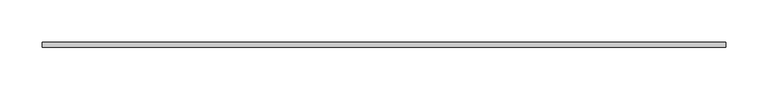
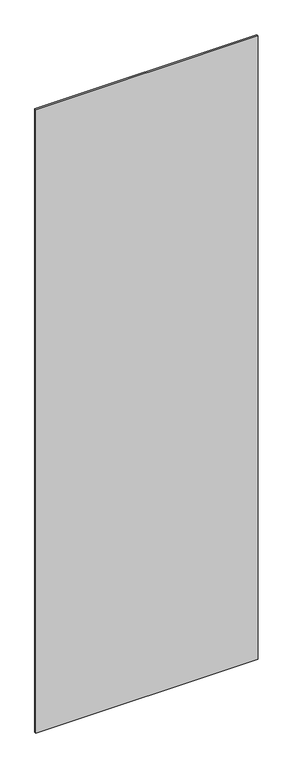
"""IFC4 building model written with IfcOpenShell, lengths in millimetres: proxy geometry, Window glass:Window glass:300352:Window glass:300352 : Window glass:Window glass:300352:300073:Window glass:300352:Window glass:300352 : Window glass:Window glass:300352:300073 : Window glass:Window glass:300352:Window glass:300352 : Window glass:Window glass:300352:300073:2 : Window glass:Window glass:300352:Window glass:300352 : Window glass:Window glass:300352:300073:Window glass:300352:Window glass:300352 : Window glass:Window glass:300352:300073 : Window glass:Window glass:300352:Window glass:300352 : Window glass:Window glass:300352:300073:300061."""

from ifc_helpers import new_model, si_unit, frame, origin, place, context, project, spatial, polyline, outline, extrude, source, transform, mapped, element, save


def generic_models_df3356e1(model_context):
    return source(origin(), model_context, "Body", "SweptSolid", [
        extrude(outline(polyline([(593690.1661787, -568062.3194464), (592877.9572692, -568062.3194464), (592877.9572692, -568055.9694464), (593690.1661787, -568055.9694464), (593690.1661787, -568062.3194464)])), frame((0.0, 0.0, 38.9089443), z_axis=(0.0, 0.0, 1.0), x_axis=(1.0, 0.0, 0.0)), (0.0, 0.0, 1.0), 2406.8704986),
    ])


if __name__ == "__main__":
    model = new_model("IFC4")
    model_context = context("Model", 3, world=origin())
    ifc_project = project(units=[si_unit("LENGTHUNIT", "METRE", prefix="MILLI")], contexts=[model_context])
    site = spatial("IfcSite", under=ifc_project)
    building = spatial("IfcBuilding", under=site)
    placement = place(None, origin())
    generic_models_shape = generic_models_df3356e1(model_context)
    element("IfcBuildingElementProxy", 1, Name="Window glass:Window glass:300352:Window glass:300352 : Window glass:Window glass:300352:300073:Window glass:300352:Window glass:300352 : Window glass:Window glass:300352:300073 : Window glass:Window glass:300352:Window glass:300352 : Window glass:Window glass:300352:300073:2 : Window glass:Window glass:300352:Window glass:300352 : Window glass:Window glass:300352:300073:Window glass:300352:Window glass:300352 : Window glass:Window glass:300352:300073 : Window glass:Window glass:300352:Window glass:300352 : Window glass:Window glass:300352:300073:300061", ObjectType="Window glass:Window glass:300352:Window glass:300352 : Window glass:Window glass:300352:300073:Window glass:300352:Window glass:300352 : Window glass:Window glass:300352:300073 : Window glass:Window glass:300352:Window glass:300352 : Window glass:Window glass:300352:300073:2 : Window glass:Window glass:300352:Window glass:300352 : Window glass:Window glass:300352:300073:Window glass:300352:Window glass:300352 : Window glass:Window glass:300352:300073 : Window glass:Window glass:300352:Window glass:300352 : Window glass:Window glass:300352:300073:300061", at=placement, inside=building, context=model_context, shape_type="MappedRepresentation", body=[
        mapped(generic_models_shape, transform((0.0, 0.0, 0.0), x_axis=(1.0, 0.0, 0.0), y_axis=(0.0, 1.0, 0.0), z_axis=(0.0, 0.0, 1.0))),
    ])
    save(model, "model.ifc")

# Revit data of these elements
# Type "Window glass:Window glass:300352:Window glass:300352 : Window glass:Window glass:300352:300073:Window glass:300352:Window glass:300352 : Window glass:Window glass:300352:300073 : Window glass:Window glass:300352:Window glass:300352 : Window glass:Window glass:300352:300073:2 : Window glass:Window glass:300352:Window glass:300352 : Window glass:Window glass:300352:300073:Window glass:300352:Window glass:300352 : Window glass:Window glass:300352:300073 : Window glass:Window glass:300352:Window glass:300352 : Window glass:Window glass:300352:300073:300061"
#   NameOverride = "Window glass:Window glass:300352:Window glass:300352 : Window glass:Window glass:300352:300073:Window glass:300352:Window glass:300352 : Window glass:Window glass:300352:300073 : Window glass:Window glass:300352:Window glass:300352 : Window glass:Window glass:300352:300073:300061"
#   ObjectTypeOverride = "Window glass:300352:Window glass:300352 : Window glass:Window glass:300352:300073 : Window glass:Window glass:300352:Window glass:300352 : Window glass:Window glass:300352:300073"
#   Reference = "Window glass"
#   Tag = "300061"
# Element 1 (IfcBuildingElementProxy, "Window glass:Window glass:300352:Window glass:300352 : Window glass:Window glass:300352:300073:Window glass:300352:Window glass:300352 : Window glass:Window glass:300352:300073 : Window glass:Window glass:300352:Window glass:300352 : Window glass:Window glass:300352:300073:2 : Window glass:Window glass:300352:Window glass:300352 : Window glass:Window glass:300352:300073:Window glass:300352:Window glass:300352 : Window glass:Window glass:300352:300073 : Window glass:Window glass:300352:Window glass:300352 : Window glass:Window glass:300352:300073:300061")
#   Materials on its faces: "SAFETY GLAZING"
# Materials
#   "SAFETY GLAZING": class "Unassigned", colour RGB 84 171 255, transparency 0, Cost = 0
